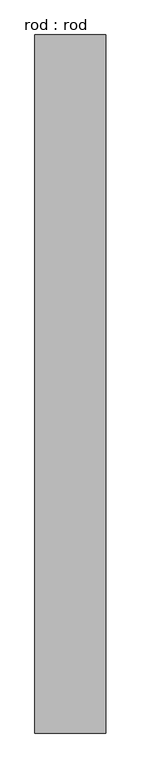
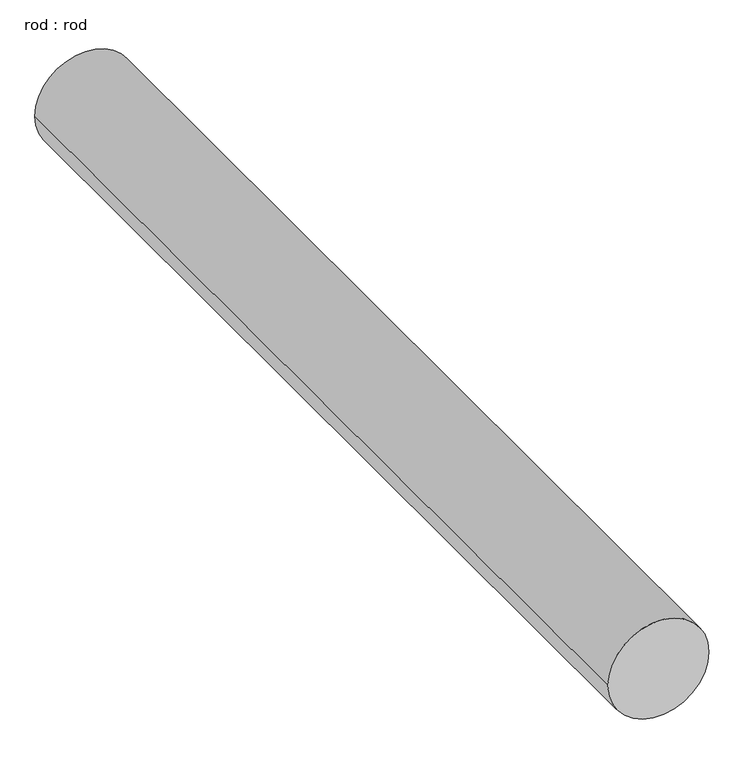
"""IFC4 building model written with IfcOpenShell, lengths in millimetres: proxy geometry, rod : rod."""

from ifc_helpers import new_model, si_unit, point, frame, frame_2d, origin, place, context, project, spatial, circle_curve, trimmed, segment, composite_curve, outline, extrude, source, transform, mapped, element, save


def rod_rod_df18659f(model_context):
    return source(origin(), model_context, "Body", "SweptSolid", [
        extrude(outline(composite_curve([segment(trimmed(circle_curve(frame_2d((0.0108462, 0.0)), 200.0), [point((0.0108462, 200.0))], [point((0.0108462, -200.0))], False, "CARTESIAN"), True, "CONTINUOUS"), segment(trimmed(circle_curve(frame_2d((0.0108462, 0.0)), 200.0), [point((0.0108462, -200.0))], [point((0.0108462, 200.0))], False, "CARTESIAN"), True, "CONTINUOUS")], self_intersect=False)), frame((0.0, 2125.5590116, 0.0), z_axis=(0.0, 1.0, 0.0), x_axis=(0.0, 0.0, 1.0)), (0.0, 0.0, 1.0), 3934.3392075),
    ])


if __name__ == "__main__":
    model = new_model("IFC4")
    model_context = context("Model", 3, world=origin())
    ifc_project = project(units=[si_unit("LENGTHUNIT", "METRE", prefix="MILLI")], contexts=[model_context])
    site = spatial("IfcSite", under=ifc_project)
    building = spatial("IfcBuilding", under=site)
    placement = place(None, origin())
    rod_rod_shape = rod_rod_df18659f(model_context)
    element("IfcBuildingElementProxy", 1, Name="rod : rod", ObjectType="rod : rod", at=placement, inside=building, context=model_context, shape_type="MappedRepresentation", body=[
        mapped(rod_rod_shape, transform((0.0, 0.0, 0.0), x_axis=(1.0, 0.0, 0.0), y_axis=(0.0, 1.0, 0.0), z_axis=(0.0, 0.0, 1.0))),
    ])
    save(model, "model.ifc")

# Revit data of these elements
# Type "rod : rod"
#   Default Elevation = 0
